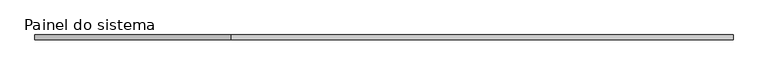
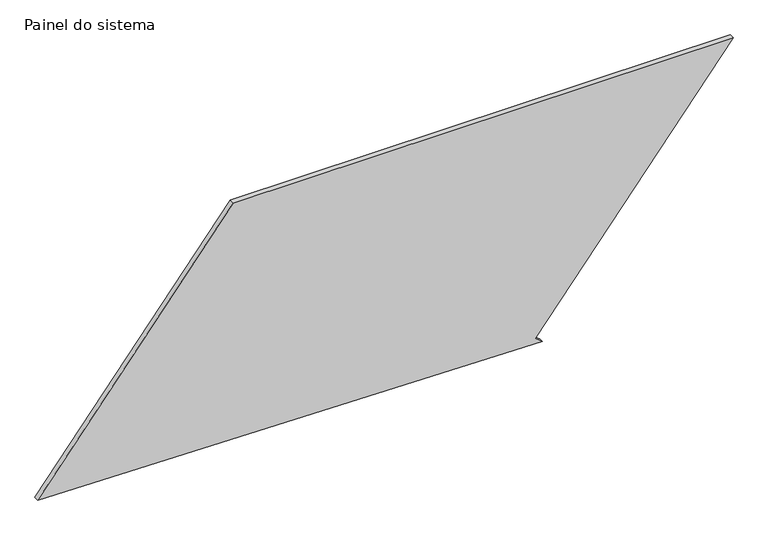
"""IFC4 building model written with IfcOpenShell, lengths in millimetres: plate geometry, Painel do sistema : Envidraçado."""

from ifc_helpers import new_model, si_unit, frame, origin, place, context, project, spatial, polyline, outline, extrude, source, transform, mapped, element, save


def painel_do_sistema_052c8021(model_context):
    return source(origin(), model_context, "Body", "SweptSolid", [
        extrude(outline(polyline([(0.0, 827.7965037), (31.1202052, 788.6617004), (1343.6641254, 1832.4036584), (1343.6641254, -801.8951278), (47.7617271, -1832.4036584), (0.0, 827.7965037)])), frame((0.0, 24.5, 0.0), z_axis=(0.0, 1.0, 0.0), x_axis=(0.0, 0.0, 1.0)), (0.0, 0.0, 1.0), 25.0),
    ])


if __name__ == "__main__":
    model = new_model("IFC4")
    model_context = context("Model", 3, world=origin())
    ifc_project = project(units=[si_unit("LENGTHUNIT", "METRE", prefix="MILLI")], contexts=[model_context])
    site = spatial("IfcSite", under=ifc_project)
    building = spatial("IfcBuilding", under=site)
    placement = place(None, origin())
    painel_do_sistema_shape = painel_do_sistema_052c8021(model_context)
    element("IfcPlate", 1, ObjectType="Painel do sistema : Envidraçado", at=placement, inside=building, context=model_context, shape_type="MappedRepresentation", body=[
        mapped(painel_do_sistema_shape, transform((0.0, 0.0, 0.0), x_axis=(1.0, 0.0, 0.0), y_axis=(0.0, 1.0, 0.0), z_axis=(0.0, 0.0, 1.0))),
    ])
    save(model, "model.ifc")

# Revit data of these elements
# Type "Painel do sistema : Envidraçado"
#   Construction Type Id = "GSP4R"
#   Analytic Construction = "Vidraça única Pilkington 1/8 pol"
#   Visual Light Transmittance = 0.9
#   Solar Heat Gain Coefficient = 0.86
#   Heat Transfer Coefficient (U) = 6.7069 W/(m²·K)
# Element 1 (IfcPlate, "Painel do sistema : Envidraçado")
#   Materials on its faces: "Vidro"
# Materials
#   "Vidro": class "Vidro", colour RGB 0 128 192, transparency 0.9, Description = "Vidro de sílica", Cost = 0
